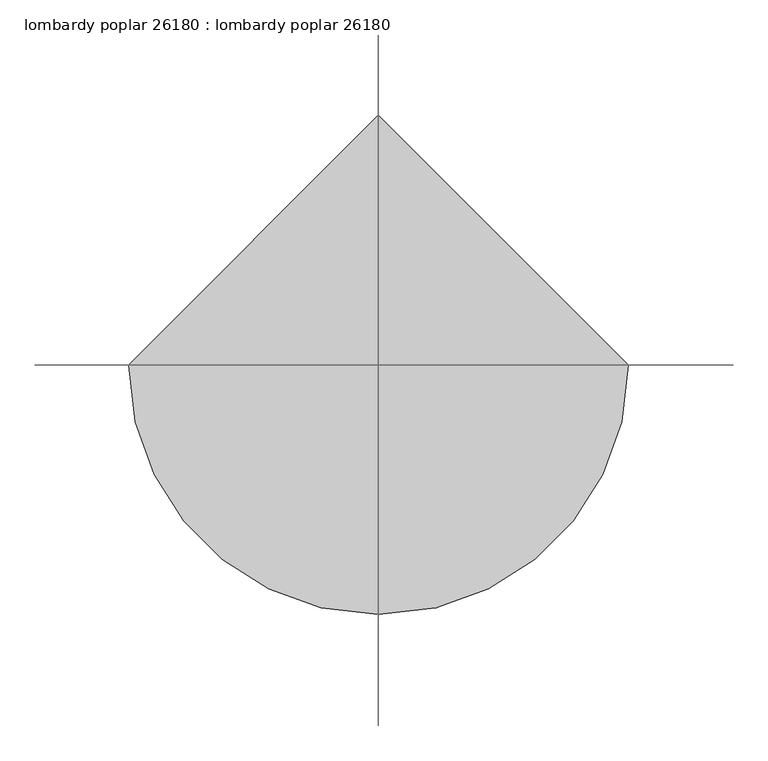
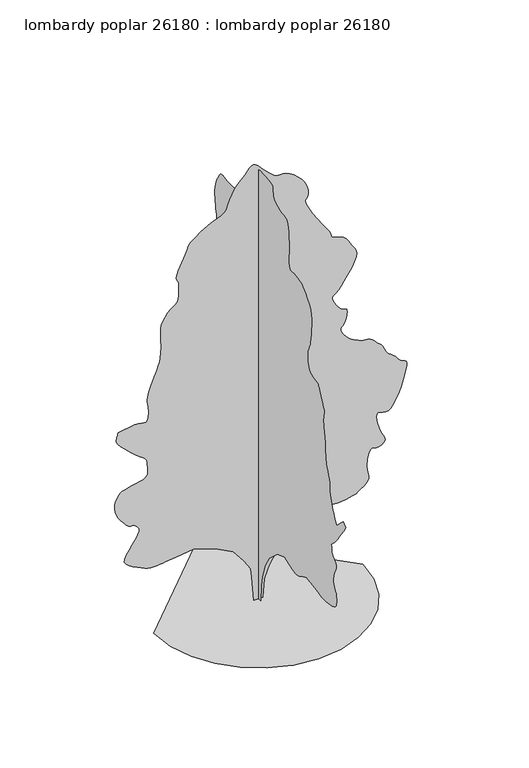
"""IFC4 building model written with IfcOpenShell, lengths in millimetres: proxy geometry, lombardy poplar 26180 : lombardy poplar 26180."""

import ifcopenshell
import ifcopenshell.guid

model = None  # the IFC model being written
_history = None  # IfcOwnerHistory: only IFC2X3 demands one
_inside = {}  # id of a spatial element -> (the spatial element, [elements in it])
_under = {}  # id of a project, library or spatial element -> (it, [spatial elements below it])
_declared = {}  # id of a project -> (the project, [libraries it declares])
_typed = {}  # id of a type object -> (the type object, [elements of that type])
_made_of = {}  # id of a material, layer set ... -> (it, [elements and type objects made of it])


def new_model(schema):
    """Start an empty IFC model of exactly this schema.

    Asked for "IFC4X3", IfcOpenShell would pick the latest addendum, in which some entities
    have other attributes; the version numbers below select the first issue.
    IFC2X3 requires an IfcOwnerHistory on every rooted entity: one is made here for all.
    """
    global model, _history
    if schema == "IFC4X3":
        model = ifcopenshell.file(schema_version=(4, 3, 0, 0))
    else:
        model = ifcopenshell.file(schema=schema)
    _inside.clear()
    _under.clear()
    _declared.clear()
    _typed.clear()
    _made_of.clear()
    _history = None
    if model.schema == "IFC2X3":
        org = make("IfcOrganization", Name="unknown")
        user = make(
            "IfcPersonAndOrganization",
            ThePerson=make("IfcPerson", FamilyName="unknown"),
            TheOrganization=org,
        )
        app = make(
            "IfcApplication",
            ApplicationDeveloper=org,
            Version="unknown",
            ApplicationFullName="unknown",
            ApplicationIdentifier="unknown",
        )
        _history = make(
            "IfcOwnerHistory",
            OwningUser=user,
            OwningApplication=app,
            ChangeAction="ADDED",
            CreationDate=0,
        )
    return model


def make(cls, **values):
    """One entity of the class cls with the attributes given. An attribute that is None is left unset."""
    return model.create_entity(
        cls, **{name: value for name, value in values.items() if value is not None}
    )


def rooted(cls, **values):
    """An entity with a GlobalId (a new one), such as an element, a storey or a relation."""
    return make(cls, GlobalId=ifcopenshell.guid.new(), OwnerHistory=_history, **values)


def si_unit(unit_type, name, prefix=None):
    """IfcSIUnit, for example si_unit("LENGTHUNIT", "METRE", prefix="MILLI")."""
    return make("IfcSIUnit", UnitType=unit_type, Prefix=prefix, Name=name)


def assignment(units):
    """IfcUnitAssignment: the units of a project."""
    return None if units is None else make("IfcUnitAssignment", Units=units)


def point(xyz):
    """IfcCartesianPoint."""
    return None if xyz is None else make("IfcCartesianPoint", Coordinates=xyz)


def direction(xyz):
    """IfcDirection."""
    return None if xyz is None else make("IfcDirection", DirectionRatios=xyz)


def frame(location, z_axis=None, x_axis=None):
    """IfcAxis2Placement3D, a coordinate frame: its origin and axes. An axis left out is left unset."""
    return make(
        "IfcAxis2Placement3D",
        Location=point(location),
        Axis=direction(z_axis),
        RefDirection=direction(x_axis),
    )


def origin():
    """The frame at (0, 0, 0) with its axes left unset."""
    return frame((0.0, 0.0, 0.0))


def place(relative_to, where):
    """IfcLocalPlacement: puts the frame where relative to a parent placement (None: the world)."""
    return make(
        "IfcLocalPlacement", PlacementRelTo=relative_to, RelativePlacement=where
    )


def context(
    kind, dimensions, precision=None, world=None, true_north=None, identifier=None
):
    """IfcGeometricRepresentationContext, for example the 3D "Model" context."""
    return make(
        "IfcGeometricRepresentationContext",
        ContextIdentifier=identifier,
        ContextType=kind,
        CoordinateSpaceDimension=dimensions,
        Precision=precision,
        WorldCoordinateSystem=world,
        TrueNorth=true_north,
    )


def project(units=None, contexts=None):
    """IfcProject with its units and contexts."""
    return rooted(
        "IfcProject",
        Name="project",
        RepresentationContexts=contexts,
        UnitsInContext=assignment(units),
    )


def spatial(cls, under=None, at=None, **own):
    """A site, building, storey or space (cls), placed at a placement, below another one or the project."""
    s = rooted(cls, ObjectPlacement=at, **own)
    if under is not None:
        _under.setdefault(under.id(), (under, []))[1].append(s)
    return s


def point_list(points):
    """IfcCartesianPointList2D or 3D."""
    cls = (
        "IfcCartesianPointList2D" if len(points[0]) == 2 else "IfcCartesianPointList3D"
    )
    return make(cls, CoordList=points)


def triangles(points, corners, closed=None, point_numbers=None):
    """IfcTriangulatedFaceSet: each triangle names its three corners, points numbered from 1."""
    return make(
        "IfcTriangulatedFaceSet",
        Coordinates=point_list(points),
        Closed=closed,
        CoordIndex=corners,
        PnIndex=point_numbers,
    )


def shape(context_of_items, identifier, shape_type, items):
    """IfcShapeRepresentation: the items that make up one representation, for example the "Body"."""
    return make(
        "IfcShapeRepresentation",
        ContextOfItems=context_of_items,
        RepresentationIdentifier=identifier,
        RepresentationType=shape_type,
        Items=items,
    )


def source(mapping_origin, context_of_items, identifier, shape_type, items):
    """IfcRepresentationMap: a shape defined once, which mapped items show again and again."""
    return make(
        "IfcRepresentationMap",
        MappingOrigin=mapping_origin,
        MappedRepresentation=shape(context_of_items, identifier, shape_type, items),
    )


def transform(
    local_origin,
    x_axis=None,
    y_axis=None,
    z_axis=None,
    scale=None,
    scale2=None,
    scale3=None,
    uniform=True,
):
    """IfcCartesianTransformationOperator3D, or its non-uniform kind. x_axis, y_axis, z_axis: its Axis1, 2, 3."""
    if uniform:
        return make(
            "IfcCartesianTransformationOperator3D",
            Axis1=direction(x_axis),
            Axis2=direction(y_axis),
            LocalOrigin=point(local_origin),
            Scale=scale,
            Axis3=direction(z_axis),
        )
    return make(
        "IfcCartesianTransformationOperator3DnonUniform",
        Axis1=direction(x_axis),
        Axis2=direction(y_axis),
        LocalOrigin=point(local_origin),
        Scale=scale,
        Axis3=direction(z_axis),
        Scale2=scale2,
        Scale3=scale3,
    )


def mapped(mapping_source, mapping_target):
    """IfcMappedItem: shows the shape of a source again, moved by a transform."""
    return make(
        "IfcMappedItem", MappingSource=mapping_source, MappingTarget=mapping_target
    )


def made_of(thing, what):
    """Note that an element or type object is made of a material, layer set ...; save() writes the relation."""
    if what is not None:
        _made_of.setdefault(what.id(), (what, []))[1].append(thing)
    return thing


def element(
    cls,
    number,
    at=None,
    inside=None,
    cuts=None,
    type_object=None,
    material=None,
    context=None,
    identifier="Body",
    shape_type=None,
    held_by="IfcProductDefinitionShape",
    body=None,
    shapes=None,
    **own,
):
    """One element of the class cls, such as IfcWall. Its Tag is "e" and its number.

    at: its placement. inside: the storey or other place that contains it. cuts: it is an
    opening in that element (IfcRelVoidsElement). A single representation is given by context,
    identifier, shape_type and body (its items); several are given by shapes. held_by: the class
    of the entity that holds the representations. save() writes the other relations.
    """
    e = rooted(cls, Tag="e%d" % number, ObjectPlacement=at, **own)
    if body is not None:
        shapes = [shape(context, identifier, shape_type, body)]
    if shapes is not None:
        e.Representation = make(held_by, Representations=shapes)
    if inside is not None:
        _inside.setdefault(inside.id(), (inside, []))[1].append(e)
    if cuts is not None:
        rooted(
            "IfcRelVoidsElement", RelatingBuildingElement=cuts, RelatedOpeningElement=e
        )
    if type_object is not None:
        _typed.setdefault(type_object.id(), (type_object, []))[1].append(e)
    return made_of(e, material)


def aggregate(whole, parts):
    """IfcRelAggregates: a whole, such as a stair, and the parts it consists of."""
    return rooted("IfcRelAggregates", RelatingObject=whole, RelatedObjects=parts)


def save(model, path):
    """Write the relations noted so far, then the file.

    IfcRelAggregates (storeys below a building ...), IfcRelContainedInSpatialStructure (elements
    in a storey), IfcRelDefinesByType, IfcRelAssociatesMaterial and IfcRelDeclares: one each for
    every whole, place, type object, material and project.
    """
    for whole, parts in _under.values():
        aggregate(whole, parts)
    for where, things in _inside.values():
        rooted(
            "IfcRelContainedInSpatialStructure",
            RelatedElements=things,
            RelatingStructure=where,
        )
    for kind, things in _typed.values():
        rooted("IfcRelDefinesByType", RelatedObjects=things, RelatingType=kind)
    for what, things in _made_of.values():
        rooted("IfcRelAssociatesMaterial", RelatedObjects=things, RelatingMaterial=what)
    for by, libraries in _declared.values():
        rooted("IfcRelDeclares", RelatingContext=by, RelatedDefinitions=libraries)
    model.write(path)


def lombardy_poplar_26180_lombardy_poplar_26180_01077960(model_context):
    return source(origin(), model_context, "Body", "Tessellation", [
        triangles([(0.0009695, 113.8156909, 0.0), (0.0009695, -104.8345258, 0.0), (0.0009695, -123.055434, 437.3009239), (0.0009695, -177.7179314, 728.8340738), (0.0009695, -323.483707, 1129.6911467), (0.0009695, -505.6928613, 1439.4461494), (0.0009695, -870.1086628, 1767.420607), (0.0009695, -1216.3049732, 1894.9664555), (0.0009695, -1398.5142002, 1822.0838402), (0.0009695, -1476.390406, 1795.1523445), (0.0009695, -1552.9941605, 1770.6083485), (0.0009695, -1627.0451637, 1750.8472), (0.0009695, -1697.2735806, 1738.2588696), (0.0009695, -1762.3991112, 1735.2286766), (0.0009695, -1821.1516296, 1744.1542946), (0.0009695, -1872.2563591, 1767.420607), (0.0009695, -1919.1091679, 1797.0624023), (0.0009695, -1965.9644474, 1823.8364948), (0.0009695, -2012.8172562, 1848.2204716), (0.0009695, -2059.6700649, 1870.6891582), (0.0009695, -2106.5227283, 1891.7279903), (0.0009695, -2153.3780079, 1911.8067066), (0.0009695, -2200.2308167, 1931.4103065), (0.0009695, -2582.8711235, 1876.7470734), (0.0009695, -2649.2156204, 1861.2353748), (0.0009695, -2715.4080917, 1846.3611374), (0.0009695, -2781.27006, 1832.7619675), (0.0009695, -2846.6750793, 1821.0754715), (0.0009695, -2911.4196739, 1811.9366398), (0.0009695, -2975.3765259, 1805.987875), (0.0009695, -3038.3939003, 1803.8619873), (0.0009695, -3111.6472778, 1806.252103), (0.0009695, -3200.5217949, 1814.0625275), (0.0009695, -3296.0764275, 1828.2459641), (0.0009695, -3389.4213112, 1849.7596218), (0.0009695, -3471.5901329, 1879.5614365), (0.0009695, -3533.6930283, 1918.6062916), (0.0009695, -3566.7892639, 1967.8516869), (0.0009695, -3579.2353065, 2021.4507408), (0.0009695, -3585.9154221, 2073.1371208), (0.0009695, -3587.8205383, 2123.2333363), (0.0009695, -3585.9154221, 2172.0521587), (0.0009695, -3581.1401321, 2219.915807), (0.0009695, -3574.4347275, 2267.139378), (0.0009695, -3566.7892639, 2314.0455265), (0.0009695, -3532.0422569, 2353.5170998), (0.0009695, -3499.7078934, 2395.5361919), (0.0009695, -3472.1235306, 2442.6555542), (0.0009695, -3451.7273918, 2497.4231415), (0.0009695, -3440.907122, 2562.3988266), (0.0009695, -3441.9992065, 2640.0972816), (0.0009695, -3457.4677391, 2733.1372421), (0.0009695, -3484.5187042, 2825.1865654), (0.0009695, -3515.3799019, 2900.6752716), (0.0009695, -3544.9708282, 2963.0830902), (0.0009695, -3568.1862717, 3015.940329), (0.0009695, -3579.9210205, 3062.7525879), (0.0009695, -3575.0695724, 3106.9993057), (0.0009695, -3548.5775848, 3152.2110809), (0.0009695, -3509.7918709, 3193.1050964), (0.0009695, -3472.6063499, 3225.0836678), (0.0009695, -3438.6212151, 3252.6171616), (0.0009695, -3409.3857903, 3280.1253662), (0.0009695, -3386.5511375, 3312.1039375), (0.0009695, -3371.6668716, 3352.997953), (0.0009695, -3366.3581841, 3407.3030685), (0.0009695, -3362.7005585, 3460.5158089), (0.0009695, -3354.9027786, 3498.4634926), (0.0009695, -3347.7145546, 3525.8699593), (0.0009695, -3345.9620453, 3547.5360786), (0.0009695, -3354.4202499, 3568.2624298), (0.0009695, -3377.8388786, 3592.7987228), (0.0009695, -3421.0188011, 3625.9458275), (0.0009695, -3481.5215034, 3679.8698616), (0.0009695, -3552.5654228, 3760.5655174), (0.0009695, -3632.3465996, 3863.5624283), (0.0009695, -3719.1381042, 3984.4155167), (0.0009695, -3811.2130074, 4118.6541252), (0.0009695, -3906.7676399, 4261.8084686), (0.0009695, -4004.1003616, 4409.432888), (0.0009695, -3894.7788368, 4518.779702), (0.0009695, -3749.0086647, 4391.221209), (0.0009695, -3603.2382019, 4227.2390671), (0.0009695, -3579.7434151, 4258.785688), (0.0009695, -3555.9689941, 4292.2630051), (0.0009695, -3531.5088593, 4329.5499733), (0.0009695, -3506.1342453, 4372.5775795), (0.0009695, -3479.4643616, 4423.2506493), (0.0009695, -3451.1939941, 4483.4992973), (0.0009695, -3421.0188011, 4555.2033508), (0.0009695, -3390.0055779, 4628.5837555), (0.0009695, -3360.2623352, 4695.8683113), (0.0009695, -3333.0587631, 4762.2383881), (0.0009695, -3309.6910034, 4832.7233299), (0.0009695, -3291.4028755, 4912.4536377), (0.0009695, -3279.5158104, 5006.5351044), (0.0009695, -3275.248629, 5120.0473618), (0.0009695, -3267.0697678, 5234.8554703), (0.0009695, -3245.5050957, 5333.3820145), (0.0009695, -3215.0252701, 5421.7481323), (0.0009695, -3180.0747871, 5505.9238083), (0.0009695, -3145.0993057, 5592.0551788), (0.0009695, -3114.6191895, 5686.1110657), (0.0009695, -3093.0545174, 5794.238768), (0.0009695, -3079.5672592, 5892.1298859), (0.0009695, -3069.8899429, 5959.4403122), (0.0009695, -3063.4130127, 6007.9286316), (0.0009695, -3059.4760437, 6049.4319122), (0.0009695, -3057.4691895, 6095.6854843), (0.0009695, -3056.7073174, 6158.5246719), (0.0009695, -3056.6055794, 6249.735965), (0.0009695, -3052.5671631, 6343.1320084), (0.0009695, -3042.1532639, 6412.2958099), (0.0009695, -3027.9291321, 6468.709227), (0.0009695, -3012.4097305, 6523.8523727), (0.0009695, -2998.1858894, 6589.2065231), (0.0009695, -2987.7716995, 6676.2017944), (0.0009695, -2983.7332832, 6796.3688782), (0.0009695, -2989.2957344, 6908.7381821), (0.0009695, -3001.5638809, 6976.78461), (0.0009695, -3013.8576073, 7018.6948425), (0.0009695, -3019.4200584, 7052.6288177), (0.0009695, -3011.6222786, 7096.7737976), (0.0009695, -2983.7332832, 7169.2908829), (0.0009695, -2929.0723755, 7288.340593), (0.0009695, -2866.7410057, 7418.1088348), (0.0009695, -2818.7857933, 7514.4256302), (0.0009695, -2782.7688057, 7582.8528488), (0.0009695, -2756.3021072, 7628.9541046), (0.0009695, -2737.0233421, 7658.3418457), (0.0009695, -2722.5201576, 7676.5535248), (0.0009695, -2710.4043274, 7689.2027527), (0.0009695, -2636.5666832, 7701.2421341), (0.0009695, -2564.8117607, 7715.3901077), (0.0009695, -2497.1818771, 7733.6523651), (0.0009695, -2435.7748695, 7758.1380798), (0.0009695, -2382.6507866, 7790.9296829), (0.0009695, -2339.8900246, 7834.0584457), (0.0009695, -2309.5548122, 7889.6335419), (0.0009695, -2289.3160767, 7951.0257248), (0.0009695, -2274.8152176, 8010.5377899), (0.0009695, -2265.0921192, 8068.4243729), (0.0009695, -2259.1968395, 8125.0662643), (0.0009695, -2256.1691174, 8180.7425171), (0.0009695, -2255.0515984, 8235.7589264), (0.0009695, -2254.8940498, 8290.4707031), (0.0009695, -2285.970932, 8345.7405853), (0.0009695, -2316.0901691, 8404.491069), (0.0009695, -2344.2968777, 8470.25159), (0.0009695, -2369.6358833, 8546.5277481), (0.0009695, -2391.1521572, 8636.8495605), (0.0009695, -2407.8857288, 8744.6726303), (0.0009695, -2418.8812786, 8873.551973), (0.0009695, -2430.0903328, 9004.9206985), (0.0009695, -2443.8493767, 9121.3031296), (0.0009695, -2453.7833633, 9227.8303482), (0.0009695, -2453.5168098, 9329.5572784), (0.0009695, -2436.6765587, 9431.5888412), (0.0009695, -2396.8874176, 9539.0561188), (0.0009695, -2327.7766651, 9657.0390335), (0.0009695, -2247.8811058, 9768.2398041), (0.0009695, -2177.228587, 9854.8798645), (0.0009695, -2111.6764835, 9921.4269653), (0.0009695, -2047.0792637, 9972.3796692), (0.0009695, -1979.2969185, 10012.156311), (0.0009695, -1904.1815907, 10045.2519653), (0.0009695, -1817.5931259, 10076.1128723), (0.0009695, -1725.5334835, 10094.8326599), (0.0009695, -1638.891679, 10096.3058258), (0.0009695, -1560.8554539, 10092.3688568), (0.0009695, -1494.6124043, 10094.8326599), (0.0009695, -1443.3501263, 10115.4325653), (0.0009695, -1410.2540359, 10166.0038971), (0.0009695, -1398.5142002, 10258.3319824), (0.0009695, -1400.4267288, 10362.6756134), (0.0009695, -1404.8895378, 10448.1971375), (0.0009695, -1409.9898079, 10525.1087219), (0.0009695, -1413.8125397, 10603.619046), (0.0009695, -1414.4501461, 10693.9414398), (0.0009695, -1409.9898079, 10806.2345856), (0.0009695, -1398.5142002, 10950.7350677), (0.0009695, -1382.6849339, 11097.4458801), (0.0009695, -1365.5779839, 11211.9737732), (0.0009695, -1345.9235149, 11297.8255096), (0.0009695, -1322.4438435, 11358.4811096), (0.0009695, -1293.8637566, 11397.4694275), (0.0009695, -1258.9083321, 11418.297226), (0.0009695, -1216.3049732, 11424.470105), (0.0009695, -1155.4822323, 11429.9813965), (0.0009695, -1073.3006933, 11446.3641174), (0.0009695, -979.6484882, 11473.2380585), (0.0009695, -884.3986336, 11510.3218414), (0.0009695, -797.4393339, 11557.2608368), (0.0009695, -728.6460766, 11613.8015717), (0.0009695, -687.9020519, 11679.5615112), (0.0009695, -672.8677952, 11749.3607391), (0.0009695, -668.0341513, 11816.289212), (0.0009695, -663.5180752, 11877.4785004), (0.0009695, -649.4413908, 11930.0811035), (0.0009695, -615.9210531, 11971.2041748), (0.0009695, -553.0790314, 11997.9757965), (0.0009695, -451.0296281, 12007.5263763), (0.0009695, -327.7864603, 12011.2087097), (0.0009695, -210.2816959, 12019.0070709), (0.0009695, -102.0189364, 12026.1694244), (0.0009695, -6.5056406, 12027.9216431), (0.0009695, 72.7523407, 12019.4895996), (0.0009695, 132.2489498, 11996.0700989), (0.0009695, 168.4781792, 11952.8657593), (0.0009695, 190.2581361, 11903.7920105), (0.0009695, 211.0820467, 11861.400412), (0.0009695, 234.4553475, 11819.0076508), (0.0009695, 263.8852554, 11769.9094849), (0.0009695, 302.8767344, 11707.4505066), (0.0009695, 354.9364746, 11624.9008942), (0.0009695, 423.5697126, 11515.57966), (0.0009695, 499.5867296, 11399.1204895), (0.0009695, 572.09851, 11297.9778259), (0.0009695, 642.0601553, 11209.5867096), (0.0009695, 710.4292379, 11131.3798553), (0.0009695, 778.1582434, 11060.8446259), (0.0009695, 846.2072874, 10995.3881561), (0.0009695, 915.531399, 10932.4978088), (0.0009695, 983.7404623, 10880.5556305), (0.0009695, 1048.444289, 10847.0786041), (0.0009695, 1110.5954372, 10828.282077), (0.0009695, 1171.1565662, 10820.3069824), (0.0009695, 1231.077618, 10819.3407623), (0.0009695, 1291.3160923, 10821.5766724), (0.0009695, 1352.8322502, 10823.1765747), (0.0009695, 1419.1287849, 10828.7646057), (0.0009695, 1490.5254444, 10841.0324615), (0.0009695, 1563.194846, 10853.3014801), (0.0009695, 1633.3164379, 10858.8639313), (0.0009695, 1697.0626923, 10851.0655701), (0.0009695, 1750.6084064, 10823.1765747), (0.0009695, 1790.1333195, 10768.5159576), (0.0009695, 1824.1844387, 10700.9526398), (0.0009695, 1861.7408672, 10636.2333344), (0.0009695, 1899.617189, 10570.5745514), (0.0009695, 1934.6234825, 10500.1404785), (0.0009695, 1963.5743317, 10421.0953033), (0.0009695, 1983.2847565, 10329.6299561), (0.0009695, 1990.5617832, 10221.8830444), (0.0009695, 1988.4357502, 10111.0130676), (0.0009695, 1982.4871307, 10010.9877777), (0.0009695, 1973.3507698, 9919.2433777), (0.0009695, 1961.6642738, 9833.2381622), (0.0009695, 1948.0651039, 9750.4350769), (0.0009695, 1933.1908665, 9668.2656738), (0.0009695, 1917.6791679, 9584.1667374), (0.0009695, 1914.3314072, 9505.3761978), (0.0009695, 1931.0649788, 9438.0663528), (0.0009695, 1961.1842159, 9378.0967575), (0.0009695, 1997.9989746, 9321.3025497), (0.0009695, 2034.813588, 9263.5682831), (0.0009695, 2064.9328251, 9200.7290955), (0.0009695, 2081.6663967, 9128.6439606), (0.0009695, 2081.1888096, 9058.6668365), (0.0009695, 2066.6854797, 9001.7964706), (0.0009695, 2041.9840805, 8953.1808334), (0.0009695, 2010.9071983, 8908.0707962), (0.0009695, 1977.2826519, 8861.6904877), (0.0009695, 1944.9307022, 8809.2646179), (0.0009695, 1917.6791679, 8745.9934799), (0.0009695, 1901.8472855, 8673.7048691), (0.0009695, 1900.361475, 8598.2164536), (0.0009695, 1911.9412914, 8520.8229218), (0.0009695, 1935.3142834, 8442.7939636), (0.0009695, 1969.2055286, 8365.374852), (0.0009695, 2012.3422852, 8289.8864365), (0.0009695, 2063.4443985, 8217.5978256), (0.0009695, 2116.1951031, 8158.060762), (0.0009695, 2166.3955273, 8113.7884644), (0.0009695, 2215.9584904, 8075.6123062), (0.0009695, 2266.796521, 8034.2101822), (0.0009695, 2320.8222931, 7980.4134659), (0.0009695, 2379.9457191, 7904.924469), (0.0009695, 2446.0820892, 7798.5239868), (0.0009695, 2515.4595406, 7684.1478287), (0.0009695, 2583.8870499, 7588.5931961), (0.0009695, 2652.6194824, 7508.3039108), (0.0009695, 2722.9518173, 7439.8511124), (0.0009695, 2796.1546165, 7379.653624), (0.0009695, 2873.4972794, 7324.2558426), (0.0009695, 2956.2759476, 7270.103334), (0.0009695, 3039.9940933, 7227.3042023), (0.0009695, 3119.5720848, 7202.0063278), (0.0009695, 3195.3148453, 7185.0137604), (0.0009695, 3267.5522964, 7167.0555542), (0.0009695, 3336.6149414, 7138.9125046), (0.0009695, 3402.807122, 7091.3130844), (0.0009695, 3466.4593414, 7015.0113464), (0.0009695, 3525.2604034, 6921.5903046), (0.0009695, 3575.4506538, 6829.7441666), (0.0009695, 3615.1508469, 6741.0728348), (0.0009695, 3642.3797081, 6657.2023727), (0.0009695, 3655.3082794, 6579.6815231), (0.0009695, 3651.9552864, 6510.1619293), (0.0009695, 3630.4414833, 6450.1673355), (0.0009695, 3590.004998, 6392.5348068), (0.0009695, 3534.6075073, 6330.4316208), (0.0009695, 3469.3295151, 6266.1192673), (0.0009695, 3399.2512344, 6201.7813339), (0.0009695, 3329.5028755, 6139.6781479), (0.0009695, 3265.1646515, 6082.0456192), (0.0009695, 3211.3676445, 6031.0934967), (0.0009695, 3161.7869499, 5985.0939789), (0.0009695, 3109.3613708, 5939.7298874), (0.0009695, 3057.8758507, 5893.4001572), (0.0009695, 3011.1906189, 5844.5304657), (0.0009695, 2973.1159081, 5791.5209106), (0.0009695, 2947.4366615, 5732.7710083), (0.0009695, 2938.0386887, 5666.680275), (0.0009695, 2934.1778778, 5597.4141541), (0.0009695, 2924.8816429, 5529.7235184), (0.0009695, 2913.6547119, 5463.0235199), (0.0009695, 2904.0535538, 5396.6025742), (0.0009695, 2899.5323181, 5329.8764145), (0.0009695, 2903.6218941, 5262.2113586), (0.0009695, 2919.8270096, 5192.9452377), (0.0009695, 2944.8458313, 5126.3719757), (0.0009695, 2972.7351173, 5066.5046997), (0.0009695, 3003.0117577, 5012.2248734), (0.0009695, 3035.1935143, 4962.3901245), (0.0009695, 3068.8231476, 4915.908078), (0.0009695, 3103.4178383, 4871.6613602), (0.0009695, 3138.4697685, 4828.5323067), (0.0009695, 3181.1415825, 4835.3141602), (0.0009695, 3222.035598, 4836.0760323), (0.0009695, 3259.4243042, 4824.696785), (0.0009695, 3291.5807716, 4795.1567276), (0.0009695, 3316.7013313, 4741.4102989), (0.0009695, 3333.0587631, 4657.3619408), (0.0009695, 3338.9008484, 4536.9916718), (0.0009695, 3338.9008484, 3935.6984322), (0.0009695, 3345.6065437, 3757.6444748), (0.0009695, 3361.2273926, 3611.1377197), (0.0009695, 3379.0582809, 3492.0371407), (0.0009695, 3392.4440918, 3396.2031647), (0.0009695, 3394.6791298, 3319.4953468), (0.0009695, 3379.0582809, 3257.747953), (0.0009695, 3338.9008484, 3206.8719887), (0.0009695, 3281.573243, 3178.2461197), (0.0009695, 3221.7053856, 3174.1568344), (0.0009695, 3163.4380119, 3176.747374), (0.0009695, 3110.9106949, 3168.187722), (0.0009695, 3068.2388809, 3130.6466995), (0.0009695, 3039.6130119, 3046.21726), (0.0009695, 3029.1482437, 2897.119384), (0.0009695, 3036.0571243, 2732.8070297), (0.0009695, 3053.1514297, 2608.9823204), (0.0009695, 3075.0460236, 2517.0268867), (0.0009695, 3096.3057724, 2448.3400909), (0.0009695, 3111.4949615, 2394.3144642), (0.0009695, 3115.2034561, 2346.3441364), (0.0009695, 3102.0208305, 2295.8261444), (0.0009695, 3089.0669701, 2254.1778145), (0.0009695, 3089.803553, 2232.6106716), (0.0009695, 3093.4355988, 2222.1992432), (0.0009695, 3089.0669701, 2214.0179111), (0.0009695, 3065.9021049, 2199.1436737), (0.0009695, 3013.0954445, 2168.6510582), (0.0009695, 2919.8270096, 2113.6169174), (0.0009695, 2822.3419716, 2052.8450455), (0.0009695, 2753.55867, 2008.9666191), (0.0009695, 2697.5010452, 1978.7940422), (0.0009695, 2638.2683235, 1959.1395733), (0.0009695, 2559.9350235, 1946.8154709), (0.0009695, 2446.5088074, 1938.6341389), (0.0009695, 2282.0948605, 1931.4103065), (0.0009695, 2105.8903542, 1933.6938881), (0.0009695, 1963.4702682, 1951.9132702), (0.0009695, 1848.4591198, 1979.6982021), (0.0009695, 1754.4869488, 2010.665934), (0.0009695, 1675.1755108, 2038.4483952), (0.0009695, 1604.1522297, 2056.670248), (0.0009695, 1535.0414772, 2058.9536842), (0.0009695, 1460.510416, 2049.0198429), (0.0009695, 1378.3312752, 2035.2631245), (0.0009695, 1289.7769421, 2018.3163391), (0.0009695, 1196.1221935, 1998.8218895), (0.0009695, 1098.6447859, 1977.4122952), (0.0009695, 998.6146271, 1954.7301041), (0.0009695, 897.3120169, 1931.4103065), (0.0009695, 532.8936719, 1639.8747585), (0.0009695, 314.2457534, 1166.1349977), (0.0009695, 168.4781792, 601.2881527), (120.1776209, 0.0005334, 0.0085345), (-116.69275, 0.0005334, 0.0085345), (-171.3552383, 0.0004849, 655.9590162), (-207.7973272, 0.0004849, 911.0508585), (-390.006209, 0.0004607, 1202.5839357), (-663.3174334, 0.0004364, 1548.7803188), (-1137.0596649, 0.0004122, 1803.8721611), (-1720.1284355, 0.0004122, 1986.078772), (-2193.8681236, 0.0004122, 1931.4180096), (-2467.1819641, 0.0004122, 1894.9766293), (-2533.7959213, 0.0004122, 1885.46689), (-2607.4327057, 0.0004122, 1874.6820831), (-2686.1473778, 0.0004122, 1865.812421), (-2768.0621452, 0.0004122, 1862.0405582), (-2851.2468933, 0.0004122, 1866.556707), (-2933.7967964, 0.0004122, 1882.5459927), (-3013.8067383, 0.0004122, 1913.1960114), (-3104.2814484, 0.0004122, 1955.5886272), (-3210.9865631, 0.0004122, 2004.6715324), (-3321.222567, 0.0004122, 2060.4522846), (-3422.2126236, 0.0004122, 2122.9234715), (-3501.2066391, 0.0003879, 2192.0875637), (-3545.4533569, 0.0003879, 2267.9445614), (-3542.2021019, 0.0003879, 2350.4969353), (-3495.1869484, 0.0003879, 2447.2326004), (-3424.930481, 0.0003879, 2559.9094437), (-3343.8031654, 0.0003637, 2679.898922), (-3264.2757523, 0.0003637, 2798.6437088), (-3198.7692856, 0.0003637, 2907.4824142), (-3159.7295174, 0.0003394, 2997.8300972), (-3159.5772011, 0.0003394, 3061.1015259), (-3182.9958298, 0.0003394, 3103.1893639), (-3206.4147491, 0.0003394, 3136.6411011), (-3229.8589577, 0.0003394, 3162.9554832), (-3253.2775864, 0.0003394, 3183.5039383), (-3276.6962151, 0.0003394, 3199.7599228), (-3300.1404236, 0.0003394, 3213.1457336), (-3323.559343, 0.0003394, 3225.1089569), (-3347.1558678, 0.0003394, 3221.5783585), (-3371.6921608, 0.0003394, 3220.486274), (-3398.1335701, 0.0003394, 3224.1438995), (-3427.4704422, 0.0003394, 3234.9897491), (-3460.6175468, 0.0003394, 3255.3858879), (-3498.5396507, 0.0003394, 3287.7199608), (-3542.2021019, 0.0003394, 3334.4304817), (-3593.6370438, 0.0003394, 3395.5174507), (-3650.1519081, 0.0003152, 3468.3897469), (-3705.7270042, 0.0003152, 3551.4730476), (-3754.2664833, 0.0003152, 3643.1668694), (-3789.7500732, 0.0003152, 3741.8713097), (-3806.1330849, 0.0002909, 3845.9855942), (-3797.2937988, 0.0002909, 3953.9354004), (-3771.4366562, 0.0002909, 4051.5730453), (-3739.8138771, 0.0002909, 4128.1791252), (-3701.2057686, 0.0002909, 4187.2342415), (-3654.2920624, 0.0002667, 4232.2937004), (-3597.828067, 0.0002667, 4266.812233), (-3530.518222, 0.0002667, 4294.3457268), (-3451.117836, 0.0002667, 4318.3486221), (-3356.8078949, 0.0002667, 4338.3131012), (-3252.3378181, 0.0002667, 4355.4326958), (-3147.5122398, 0.0002667, 4375.7270966), (-3052.2622398, 0.0002667, 4405.2674446), (-2976.4689011, 0.0002667, 4450.0981384), (-2929.9868546, 0.0002667, 4516.2906097), (-2922.6971832, 0.0002667, 4609.8895477), (-2933.5936111, 0.0002425, 4707.6283493), (-2938.4197701, 0.0002425, 4784.9713028), (-2942.3058701, 0.0002425, 4846.0582718), (-2950.332415, 0.0002425, 4895.0291199), (-2967.578746, 0.0002425, 4936.0504532), (-2999.2018158, 0.0002425, 4973.2359741), (-3050.2556763, 0.0002425, 5010.7517075), (-3135.4978569, 0.0002182, 5072.041571), (-3254.8777794, 0.0002182, 5168.7141586), (-3391.1232422, 0.0002182, 5287.0778641), (-3527.0637817, 0.0002182, 5413.3916656), (-3645.4783562, 0.000194, 5533.9906998), (-3729.1459236, 0.000194, 5635.1333633), (-3760.8704407, 0.000194, 5703.129213), (-3759.2702477, 0.000194, 5747.3247711), (-3754.799881, 0.000194, 5786.7456207), (-3747.9418694, 0.000194, 5822.178923), (-3739.1787415, 0.0001697, 5854.4112579), (-3728.9933167, 0.0001697, 5884.2815277), (-3717.8428345, 0.0001697, 5912.5263153), (-3706.2095329, 0.0001697, 5940.0089401), (-3268.8984352, 0.0001697, 6012.8818176), (-3174.1312546, 0.0001697, 6014.48172), (-3093.0545174, 0.0001697, 5998.8605804), (-3026.0240158, 0.0001697, 5982.2743835), (-2973.319384, 0.0001697, 5981.0046936), (-2935.2955421, 0.0001697, 6011.2813339), (-2912.232415, 0.0001697, 6089.3864502), (-2904.4852135, 0.0001697, 6231.5242859), (-2910.9624344, 0.0001455, 6377.1421417), (-2925.0848282, 0.0001455, 6470.4870255), (-2938.9022987, 0.0001455, 6535.1301727), (-2944.4394608, 0.0001455, 6594.6678177), (-2933.6953491, 0.0001212, 6672.7217743), (-2898.7448662, 0.0001212, 6792.8126999), (-2831.5873375, 0.0001212, 6978.5879883), (-2754.346122, 9.7e-05, 7175.5649185), (-2693.3861801, 9.7e-05, 7325.0435852), (-2647.0567406, 9.7e-05, 7444.2456116), (-2613.8081886, 7.27e-05, 7550.3920395), (-2592.0150421, 7.27e-05, 7660.678331), (-2580.127977, 7.27e-05, 7792.3011108), (-2576.4956406, 4.85e-05, 7962.5064194), (-2580.0009499, 4.85e-05, 8135.9626923), (-2586.7063545, 4.85e-05, 8272.4363388), (-2590.8467995, 2.42e-05, 8381.8087326), (-2586.7063545, 2.42e-05, 8473.985083), (-2568.5455444, 2.42e-05, 8558.8211838), (-2530.6106506, 2.42e-05, 8646.1972458), (-2467.1819641, 0.0, 8746.0190598), (-2393.5550629, 0.0, 8838.8046753), (-2328.8511635, 0.0, 8903.8797729), (-2273.0728821, 0.0, 8949.1932861), (-2226.2200733, 0.0, 8982.7208908), (-2188.2902664, 0.0, 9012.4138458), (-2159.2860775, 0.0, 9046.2460831), (-2139.2048904, 0.0, 9092.1950226), (-2125.7124001, -2.42e-05, 9135.3493652), (-2116.0452576, -2.42e-05, 9162.8575699), (-2109.5630951, -2.42e-05, 9185.920697), (-2105.6338291, -2.42e-05, 9215.6642303), (-2103.6144756, -2.42e-05, 9263.2636505), (-2102.8701897, -2.42e-05, 9339.8700211), (-2102.7661263, -2.42e-05, 9456.6332428), (-2113.0708752, -4.85e-05, 9567.5549606), (-2136.1264446, -4.85e-05, 9634.4840149), (-2160.137043, -4.85e-05, 9680.3817947), (-2173.3094948, -4.85e-05, 9728.1846909), (-2163.855566, -4.85e-05, 9800.8540924), (-2119.9745235, -7.27e-05, 9921.3258087), (-2029.8808949, -7.27e-05, 10112.5618103), (-1939.4672276, -7.27e-05, 10305.830246), (-1888.8958958, -9.7e-05, 10431.5097839), (-1857.7656738, -9.7e-05, 10511.3165405), (-1825.6805683, -9.7e-05, 10566.8654755), (-1772.2389175, -9.7e-05, 10619.9006104), (-1677.0450188, -9.7e-05, 10692.0369049), (-1519.6973557, -0.0001212, 10804.9648956), (-1341.6868549, -0.0001212, 10917.309201), (-1195.5481733, -0.0001212, 10985.3806274), (-1077.4586517, -0.0001212, 11027.29086), (-983.5905441, -0.0001212, 11061.2248352), (-910.1237349, -0.0001212, 11105.3698151), (-853.2303326, -0.0001455, 11177.8874817), (-809.0852074, -0.0001455, 11296.9371918), (-759.9464916, -0.0001455, 11440.4714539), (-694.8717573, -0.0001697, 11572.8563965), (-620.2365601, -0.0001697, 11691.8293671), (-542.413585, -0.0001697, 11795.2079407), (-467.775808, -0.0001697, 11880.7294647), (-402.7036534, -0.0001697, 11946.1847717), (-353.5649014, -0.000194, 11989.3146973), (-315.2642959, -0.000194, 12029.8529205), (-276.9611651, -0.000194, 12081.541626), (-236.4299363, -0.000194, 12133.2303314), (-191.4351718, -0.000194, 12173.7685547), (-139.7475292, -0.000194, 12191.9802338), (-79.1353495, -0.000194, 12176.7404663), (-7.3676139, -0.000194, 12116.8731903), (68.4904824, -0.000194, 12035.3130524), (139.8862108, -0.000194, 11962.0605469), (206.8199341, -0.0001697, 11896.4517609), (269.290376, -0.0001697, 11837.8797546), (327.3013518, -0.0001697, 11785.6573608), (380.8469934, -0.0001697, 11739.1753143), (429.9324057, -0.0001697, 11697.7987701), (477.3160323, -0.0001697, 11672.4491547), (527.8899076, -0.0001697, 11666.8622864), (584.8366133, -0.0001697, 11669.5795624), (651.343891, -0.0001697, 11669.0970337), (730.6019165, -0.0001697, 11653.9584229), (825.7958879, -0.0001697, 11612.684198), (940.1160175, -0.0001455, 11533.7913391), (1053.1051964, -0.0001455, 11434.3508972), (1143.4680674, -0.0001455, 11338.4148926), (1213.1096741, -0.0001455, 11245.0194305), (1263.9477047, -0.0001455, 11153.2238708), (1297.8921444, -0.0001212, 11062.0631561), (1316.8558125, -0.0001212, 10970.5978088), (1322.7537083, -0.0001212, 10877.8371918), (1310.6404942, -0.0001212, 10807.3019623), (1283.8688725, -0.0001212, 10768.6426941), (1256.7747414, -0.0001212, 10740.1444336), (1243.7064983, -9.7e-05, 10700.2154755), (1259.0074539, -9.7e-05, 10627.1141235), (1317.0158318, -9.7e-05, 10499.1998383), (1432.0777039, -7.27e-05, 10294.7809204), (1568.3356659, -7.27e-05, 10074.4362305), (1681.0074223, -4.85e-05, 9906.365094), (1771.0503273, -4.85e-05, 9780.3565063), (1839.4167938, -4.85e-05, 9686.22388), (1887.067083, -4.85e-05, 9613.757373), (1914.9562237, -4.85e-05, 9552.772142), (1924.041861, -2.42e-05, 9493.0571823), (1943.5896503, -2.42e-05, 9444.2892288), (1995.6494087, -2.42e-05, 9415.2822784), (2070.3380184, -2.42e-05, 9394.5812164), (2157.7773033, -2.42e-05, 9370.6797684), (2248.0842911, -2.42e-05, 9332.0972397), (2331.3809509, -2.42e-05, 9267.4035141), (2397.7841652, -2.42e-05, 9165.0928986), (2454.6240097, 0.0, 9055.2379761), (2511.1467224, 0.0, 8968.9542892), (2560.341394, 0.0, 8896.3866257), (2595.190139, 0.0, 8827.6541931), (2608.6773972, 0.0, 8752.8512009), (2593.7931313, 2.42e-05, 8662.1230179), (2543.5520119, 2.42e-05, 8545.5876892), (2481.3447624, 2.42e-05, 8432.1260101), (2431.8886242, 2.42e-05, 8349.5508179), (2390.080275, 2.42e-05, 8286.457576), (2350.8220608, 4.85e-05, 8231.3138489), (2309.0163277, 4.85e-05, 8172.6656845), (2259.5600441, 4.85e-05, 8099.0312256), (2197.3530853, 4.85e-05, 7998.9553574), (2127.0206051, 4.85e-05, 7904.0355698), (2060.8307499, 7.27e-05, 7844.1677124), (2005.159148, 7.27e-05, 7805.3311295), (1966.378521, 7.27e-05, 7773.5051651), (1950.8666771, 7.27e-05, 7734.6685822), (1964.9992447, 7.27e-05, 7674.8007248), (2015.1464745, 7.27e-05, 7579.8815186), (2080.6452381, 7.27e-05, 7478.1545883), (2137.5387131, 9.7e-05, 7404.1387573), (2187.2590794, 9.7e-05, 7353.262793), (2231.2468014, 9.7e-05, 7320.852562), (2270.9265015, 9.7e-05, 7302.3106705), (2307.7412601, 9.7e-05, 7293.0141449), (2343.1207867, 9.7e-05, 7288.340593), (2346.839455, 9.7e-05, 7260.6544922), (2349.4429298, 9.7e-05, 7230.9109589), (2349.8136921, 9.7e-05, 7197.027562), (2346.839455, 9.7e-05, 7156.9212891), (2339.4022636, 9.7e-05, 7108.5341263), (2326.3873604, 0.0001212, 7049.7842239), (2306.6795517, 0.0001212, 6978.5879883), (2277.832766, 0.0001212, 6914.427951), (2243.2507198, 0.0001212, 6871.273027), (2210.5813477, 0.0001212, 6838.9901138), (2187.4724384, 0.0001212, 6807.3158844), (2181.5771587, 0.0001212, 6766.0922379), (2200.5406815, 0.0001212, 6705.1064255), (2252.0163185, 0.0001455, 6614.1747665), (2322.1379105, 0.0001455, 6519.5090332), (2391.3020027, 0.0001455, 6450.3452316), (2458.553421, 0.0001455, 6400.9424332), (2522.9372818, 0.0001455, 6365.5602905), (2583.5059685, 0.0001455, 6338.4584564), (2639.2842499, 0.0001455, 6313.9221634), (2689.322184, 0.0001455, 6286.184903), (2738.2427444, 0.0001455, 6263.7822006), (2790.6680328, 0.0001455, 6254.1048843), (2845.659153, 0.0001697, 6249.8632828), (2902.2248863, 0.0001697, 6243.6909851), (2959.4507538, 0.0001697, 6228.2989014), (3016.3466995, 0.0001697, 6196.3200394), (3071.9473755, 0.0001697, 6140.4403107), (3121.4519119, 0.0001697, 6084.0774719), (3162.3712166, 0.0001697, 6048.746489), (3197.2199615, 0.0001697, 6024.2607742), (3228.5633972, 0.0001697, 6000.4104858), (3258.9417755, 0.0001697, 5966.9840378), (3290.9203468, 0.0001697, 5913.8215851), (3327.0390724, 0.000194, 5830.687706), (3367.3235321, 0.000194, 5746.3091354), (3410.4525856, 0.000194, 5689.0573975), (3457.0869484, 0.000194, 5648.0366455), (3507.8614655, 0.000194, 5612.4510269), (3563.4365616, 0.000194, 5571.430275), (3624.4217926, 0.000194, 5514.178537), (3691.4522942, 0.0002182, 5429.8255463), (3759.9306725, 0.0002182, 5354.920816), (3822.0335678, 0.0002182, 5319.208461), (3873.620826, 0.0002182, 5301.6827866), (3910.5270035, 0.0002182, 5281.2863571), (3928.6625244, 0.0002182, 5236.989061), (3923.8110764, 0.0002182, 5147.7334625), (3891.883374, 0.0002425, 4992.5144485), (3839.8897453, 0.0002425, 4801.4304726), (3779.2600159, 0.0002667, 4621.8274818), (3712.6105957, 0.0002667, 4458.4801849), (3642.4302864, 0.0002667, 4316.1641624), (3571.3104996, 0.0002909, 4199.6799934), (3501.7653259, 0.0002909, 4113.777388), (3436.3605972, 0.0002909, 4063.2569252), (3368.5935127, 0.0002909, 4052.055574), (3295.6956367, 0.0002909, 4067.2956322), (3225.9981468, 0.0002909, 4088.6059593), (3167.7813515, 0.0002909, 4095.5657089), (3129.3258499, 0.0002909, 4067.7781609), (3118.9119507, 0.0002909, 3984.8471764), (3144.8452515, 0.0002909, 3826.3769073), (3196.8388802, 0.0003152, 3648.5264259), (3252.998243, 0.0003152, 3514.6686081), (3304.0521034, 0.0003152, 3415.2278755), (3340.7550957, 0.0003394, 3340.6280685), (3353.8615631, 0.0003394, 3281.3444778), (3334.1764275, 0.0003394, 3227.8015251), (3272.3784554, 0.0003394, 3170.4230507), (3191.911274, 0.0003394, 3134.2534561), (3121.6295174, 0.0003394, 3135.3711205), (3060.5934174, 0.0003394, 3150.839653), (3007.8379166, 0.0003394, 3157.6976646), (2962.4226654, 0.0003394, 3132.9834755), (2923.3828972, 0.0003394, 3053.7862747), (2889.7532639, 0.0003637, 2897.119384), (2876.0881096, 0.0003637, 2719.1165863), (2887.6196732, 0.0003879, 2584.1155243), (2909.3366615, 0.0003879, 2481.6546272), (2926.3039398, 0.0003879, 2401.1749466), (2923.4846352, 0.0003879, 2332.1708736), (2885.9180328, 0.0003879, 2264.1218296), (2798.6437088, 0.0003879, 2186.5098518), (2701.5906212, 0.0004122, 2115.113047), (2635.7792313, 0.0004122, 2068.2602383), (2587.7987297, 0.0004122, 2039.2560493), (2544.2885948, 0.0004122, 2021.4075748), (2491.8603996, 0.0004122, 2008.0191479), (2417.1185955, 0.0004122, 1992.4007698), (2306.6795517, 0.0004122, 1967.8592445), (2182.1079403, 0.0004122, 1946.8763683), (2070.9247559, 0.0004122, 1942.7844669), (1968.6644279, 0.0004122, 1950.1707893), (1870.8670544, 0.0004122, 1963.60994), (1773.0695354, 0.0004122, 1977.6865517), (1670.8093529, 0.0004122, 1986.9829319), (1559.6260231, 0.0004122, 1986.078772), (1454.709026, 0.0004122, 1976.1447853), (1371.7857445, 0.0004122, 1962.3882122), (1307.1885246, 0.0004122, 1945.4412815), (1257.2547993, 0.0004122, 1925.9468319), (1218.3166964, 0.0004122, 1904.5372375), (1186.70896, 0.0004122, 1881.8550465), (1158.7664795, 0.0004122, 1858.5353943), (1158.4464409, 0.0004364, 1761.2688023), (1156.2163445, 0.0004364, 1666.0722874), (1150.1584293, 0.0004364, 1575.0234844), (1138.3677246, 0.0004364, 1490.1876743), (1118.9240713, 0.0004364, 1413.6372597), (1089.9198824, 0.0004607, 1347.4475498), (1049.4399405, 0.0004607, 1293.6884766), (1004.179767, 0.0004607, 1251.6160446), (961.7897673, 0.0004607, 1218.1490467), (921.7874125, 0.0004607, 1191.8550121), (883.7001297, 0.0004607, 1171.2962379), (847.045463, 0.0004607, 1155.0403261), (811.3483686, 0.0004607, 1141.6519718), (776.1287888, 0.0004607, 1129.7013205), (466.3737496, 0.0004607, 1129.7013205), (284.1645772, 0.0004849, 856.3875526), (156.6199641, 0.0005092, 510.1912059), (-2766.0555817, 0.0, 0.0100862), (-2692.9292313, -633.8001217, 0.0100862), (-2484.680024, -1215.8427195, 0.0100862), (-2157.9602863, -1729.4553371, 0.0100862), (-1729.4553371, -2157.9602863, 0.0100862), (-1215.8427195, -2484.680024, 0.0100862), (-633.8001217, -2692.9292313, 0.0100862), (0.0001209, -2766.0555817, 0.0100862), (633.8001217, -2692.9292313, 0.0100862), (1215.8427195, -2484.680024, 0.0100862), (1729.4553371, -2157.9602863, 0.0100862), (2157.9602863, -1729.4553371, 0.0100862), (2484.680024, -1215.8427195, 0.0100862), (2692.9292313, -633.8001217, 0.0100862), (2766.0555817, 0.0002425, 0.0100862), (-0.0003627, 2766.0555817, 0.0100862)], [[1, 2, 3], [388, 1, 3], [388, 3, 4], [387, 388, 4], [387, 4, 5], [80, 81, 82], [79, 80, 82], [79, 82, 83], [78, 79, 83], [77, 78, 83], [387, 5, 6], [386, 387, 6], [76, 77, 83], [386, 6, 7], [359, 360, 361], [359, 361, 362], [385, 386, 7], [75, 76, 83], [75, 83, 84], [75, 84, 85], [74, 75, 85], [73, 74, 85], [73, 85, 86], [72, 73, 86], [72, 86, 87], [358, 359, 362], [358, 362, 363], [72, 87, 88], [131, 132, 133], [71, 72, 88], [130, 131, 133], [129, 130, 133], [71, 88, 89], [44, 45, 46], [128, 129, 133], [71, 89, 90], [207, 208, 209], [207, 209, 210], [206, 207, 210], [205, 206, 210], [205, 210, 211], [205, 211, 212], [204, 205, 212], [204, 212, 213], [203, 204, 213], [203, 213, 214], [203, 214, 215], [202, 203, 215], [202, 215, 216], [201, 202, 216], [200, 201, 216], [199, 200, 216], [198, 199, 216], [197, 198, 216], [196, 197, 216], [195, 196, 216], [194, 195, 216], [194, 216, 217], [193, 194, 217], [193, 217, 218], [193, 218, 219], [192, 193, 219], [192, 219, 220], [191, 192, 220], [191, 220, 221], [191, 221, 222], [190, 191, 222], [190, 222, 223], [128, 133, 134], [127, 128, 134], [71, 90, 91], [235, 236, 237], [234, 235, 237], [233, 234, 237], [233, 237, 238], [232, 233, 238], [232, 238, 239], [231, 232, 239], [231, 239, 240], [231, 240, 241], [231, 241, 242], [230, 231, 242], [230, 242, 243], [230, 243, 244], [230, 244, 245], [229, 230, 245], [229, 245, 246], [228, 229, 246], [228, 246, 247], [227, 228, 247], [227, 247, 248], [227, 248, 249], [226, 227, 249], [226, 249, 250], [226, 250, 251], [225, 226, 251], [225, 251, 252], [224, 225, 252], [71, 91, 92], [189, 190, 223], [330, 331, 332], [330, 332, 333], [329, 330, 333], [329, 333, 334], [328, 329, 334], [328, 334, 335], [328, 335, 336], [327, 328, 336], [385, 7, 8], [342, 343, 344], [341, 342, 344], [341, 344, 345], [340, 341, 345], [340, 345, 346], [339, 340, 346], [339, 346, 347], [338, 339, 347], [337, 338, 347], [337, 347, 348], [336, 337, 348], [327, 336, 348], [326, 327, 348], [325, 326, 348], [324, 325, 348], [323, 324, 348], [126, 127, 134], [126, 134, 135], [357, 358, 363], [357, 363, 364], [356, 357, 364], [355, 356, 364], [354, 355, 364], [353, 354, 364], [353, 364, 365], [352, 353, 365], [352, 365, 366], [352, 366, 367], [352, 367, 368], [352, 368, 369], [352, 369, 370], [351, 352, 370], [351, 370, 371], [351, 371, 372], [350, 351, 372], [350, 372, 373], [350, 373, 374], [350, 374, 375], [350, 375, 376], [349, 350, 376], [349, 376, 377], [348, 349, 377], [323, 348, 377], [323, 377, 378], [323, 378, 379], [323, 379, 380], [322, 323, 380], [322, 380, 381], [322, 381, 382], [321, 322, 382], [321, 382, 383], [321, 383, 384], [321, 384, 385], [321, 385, 8], [320, 321, 8], [319, 320, 8], [318, 319, 8], [317, 318, 8], [316, 317, 8], [315, 316, 8], [314, 315, 8], [313, 314, 8], [57, 58, 59], [56, 57, 59], [56, 59, 60], [55, 56, 60], [55, 60, 61], [54, 55, 61], [54, 61, 62], [53, 54, 62], [53, 62, 63], [53, 63, 64], [52, 53, 64], [36, 37, 38], [36, 38, 39], [35, 36, 39], [35, 39, 40], [35, 40, 41], [34, 35, 41], [34, 41, 42], [34, 42, 43], [33, 34, 43], [33, 43, 44], [33, 44, 46], [33, 46, 47], [32, 33, 47], [32, 47, 48], [31, 32, 48], [30, 31, 48], [30, 48, 49], [29, 30, 49], [28, 29, 49], [27, 28, 49], [26, 27, 49], [26, 49, 50], [25, 26, 50], [24, 25, 50], [24, 50, 51], [23, 24, 51], [23, 51, 52], [23, 52, 64], [23, 64, 65], [23, 65, 66], [23, 66, 67], [23, 67, 68], [23, 68, 69], [23, 69, 70], [22, 23, 70], [21, 22, 70], [20, 21, 70], [19, 20, 70], [18, 19, 70], [125, 126, 135], [125, 135, 136], [189, 223, 224], [189, 224, 252], [189, 252, 253], [188, 189, 253], [187, 188, 253], [186, 187, 253], [185, 186, 253], [184, 185, 253], [183, 184, 253], [182, 183, 253], [181, 182, 253], [180, 181, 253], [179, 180, 253], [178, 179, 253], [177, 178, 253], [176, 177, 253], [175, 176, 253], [174, 175, 253], [173, 174, 253], [172, 173, 253], [172, 253, 254], [172, 254, 255], [172, 255, 256], [172, 256, 257], [172, 257, 258], [172, 258, 259], [172, 259, 260], [172, 260, 261], [172, 261, 262], [172, 262, 263], [172, 263, 264], [172, 264, 265], [172, 265, 266], [172, 266, 267], [172, 267, 268], [172, 268, 269], [171, 172, 269], [171, 269, 270], [171, 270, 271], [170, 171, 271], [170, 271, 272], [169, 170, 272], [168, 169, 272], [167, 168, 272], [166, 167, 272], [165, 166, 272], [164, 165, 272], [163, 164, 272], [162, 163, 272], [161, 162, 272], [160, 161, 272], [159, 160, 272], [158, 159, 272], [157, 158, 272], [156, 157, 272], [155, 156, 272], [154, 155, 272], [153, 154, 272], [152, 153, 272], [151, 152, 272], [150, 151, 272], [149, 150, 272], [148, 149, 272], [147, 148, 272], [146, 147, 272], [145, 146, 272], [144, 145, 272], [143, 144, 272], [142, 143, 272], [141, 142, 272], [140, 141, 272], [139, 140, 272], [138, 139, 272], [138, 272, 273], [138, 273, 274], [137, 138, 274], [137, 274, 275], [137, 275, 276], [137, 276, 277], [137, 277, 278], [137, 278, 279], [137, 279, 280], [137, 280, 281], [137, 281, 282], [137, 282, 283], [136, 137, 283], [125, 136, 283], [124, 125, 283], [123, 124, 283], [122, 123, 283], [121, 122, 283], [120, 121, 283], [119, 120, 283], [118, 119, 283], [117, 118, 283], [116, 117, 283], [115, 116, 283], [114, 115, 283], [113, 114, 283], [112, 113, 283], [111, 112, 283], [110, 111, 283], [109, 110, 283], [108, 109, 283], [107, 108, 283], [106, 107, 283], [105, 106, 283], [104, 105, 283], [103, 104, 283], [103, 283, 284], [102, 103, 284], [102, 284, 285], [101, 102, 285], [100, 101, 285], [99, 100, 285], [98, 99, 285], [97, 98, 285], [96, 97, 285], [95, 96, 285], [94, 95, 285], [94, 285, 286], [93, 94, 286], [93, 286, 287], [92, 93, 287], [71, 92, 287], [70, 71, 287], [18, 70, 287], [17, 18, 287], [16, 17, 287], [15, 16, 287], [14, 15, 287], [13, 14, 287], [12, 13, 287], [11, 12, 287], [10, 11, 287], [9, 10, 287], [8, 9, 287], [313, 8, 287], [312, 313, 287], [311, 312, 287], [310, 311, 287], [309, 310, 287], [308, 309, 287], [307, 308, 287], [306, 307, 287], [305, 306, 287], [305, 287, 288], [304, 305, 288], [304, 288, 289], [303, 304, 289], [303, 289, 290], [303, 290, 291], [303, 291, 292], [303, 292, 293], [303, 293, 294], [303, 294, 295], [302, 303, 295], [302, 295, 296], [302, 296, 297], [301, 302, 297], [301, 297, 298], [300, 301, 298], [300, 298, 299], [745, 389, 390], [745, 390, 391], [744, 745, 391], [744, 391, 392], [622, 623, 624], [743, 744, 392], [743, 392, 393], [474, 475, 476], [473, 474, 476], [472, 473, 476], [471, 472, 476], [470, 471, 476], [469, 470, 476], [468, 469, 476], [467, 468, 476], [466, 467, 476], [465, 466, 476], [464, 465, 476], [464, 476, 477], [464, 477, 478], [464, 478, 479], [463, 464, 479], [463, 479, 480], [462, 463, 480], [461, 462, 480], [460, 461, 480], [460, 480, 481], [743, 393, 394], [622, 624, 625], [459, 460, 481], [621, 622, 625], [621, 625, 626], [621, 626, 627], [668, 669, 670], [668, 670, 671], [667, 668, 671], [667, 671, 672], [666, 667, 672], [620, 621, 627], [620, 627, 628], [620, 628, 629], [666, 672, 673], [620, 629, 630], [619, 620, 630], [619, 630, 631], [619, 631, 632], [619, 632, 633], [618, 619, 633], [618, 633, 634], [665, 666, 673], [550, 551, 552], [550, 552, 553], [549, 550, 553], [548, 549, 553], [548, 553, 554], [547, 548, 554], [547, 554, 555], [546, 547, 555], [545, 546, 555], [545, 555, 556], [544, 545, 556], [543, 544, 556], [543, 556, 557], [542, 543, 557], [542, 557, 558], [541, 542, 558], [541, 558, 559], [540, 541, 559], [539, 540, 559], [539, 559, 560], [538, 539, 560], [538, 560, 561], [617, 618, 634], [690, 691, 692], [690, 692, 693], [689, 690, 693], [689, 693, 694], [689, 694, 695], [689, 695, 696], [688, 689, 696], [688, 696, 697], [687, 688, 697], [687, 697, 698], [686, 687, 698], [410, 411, 412], [410, 412, 413], [409, 410, 413], [408, 409, 413], [408, 413, 414], [407, 408, 414], [407, 414, 415], [406, 407, 415], [406, 415, 416], [405, 406, 416], [404, 405, 416], [403, 404, 416], [402, 403, 416], [401, 402, 416], [400, 401, 416], [400, 416, 417], [399, 400, 417], [398, 399, 417], [397, 398, 417], [397, 417, 418], [396, 397, 418], [396, 418, 419], [665, 673, 674], [664, 665, 674], [663, 664, 674], [662, 663, 674], [661, 662, 674], [661, 674, 675], [661, 675, 676], [660, 661, 676], [660, 676, 677], [660, 677, 678], [660, 678, 679], [660, 679, 680], [660, 680, 681], [660, 681, 682], [660, 682, 683], [659, 660, 683], [659, 683, 684], [658, 659, 684], [537, 538, 561], [657, 658, 684], [656, 657, 684], [655, 656, 684], [654, 655, 684], [653, 654, 684], [652, 653, 684], [651, 652, 684], [650, 651, 684], [649, 650, 684], [648, 649, 684], [647, 648, 684], [646, 647, 684], [645, 646, 684], [644, 645, 684], [643, 644, 684], [642, 643, 684], [641, 642, 684], [640, 641, 684], [639, 640, 684], [537, 561, 562], [638, 639, 684], [704, 705, 706], [704, 706, 707], [703, 704, 707], [703, 707, 708], [702, 703, 708], [702, 708, 709], [702, 709, 710], [702, 710, 711], [702, 711, 712], [702, 712, 713], [701, 702, 713], [701, 713, 714], [701, 714, 715], [701, 715, 716], [701, 716, 717], [701, 717, 718], [700, 701, 718], [700, 718, 719], [700, 719, 720], [699, 700, 720], [699, 720, 721], [699, 721, 722], [698, 699, 722], [686, 698, 722], [685, 686, 722], [685, 722, 723], [685, 723, 724], [684, 685, 724], [638, 684, 724], [638, 724, 725], [637, 638, 725], [637, 725, 726], [637, 726, 727], [636, 637, 727], [636, 727, 728], [635, 636, 728], [574, 575, 576], [458, 459, 481], [396, 419, 420], [574, 576, 577], [573, 574, 577], [572, 573, 577], [571, 572, 577], [570, 571, 577], [569, 570, 577], [568, 569, 577], [568, 577, 578], [567, 568, 578], [566, 567, 578], [565, 566, 578], [564, 565, 578], [563, 564, 578], [562, 563, 578], [537, 562, 578], [537, 578, 579], [537, 579, 580], [536, 537, 580], [536, 580, 581], [536, 581, 582], [535, 536, 582], [534, 535, 582], [533, 534, 582], [532, 533, 582], [531, 532, 582], [530, 531, 582], [529, 530, 582], [528, 529, 582], [527, 528, 582], [526, 527, 582], [525, 526, 582], [524, 525, 582], [523, 524, 582], [522, 523, 582], [521, 522, 582], [520, 521, 582], [519, 520, 582], [518, 519, 582], [517, 518, 582], [516, 517, 582], [515, 516, 582], [515, 582, 583], [514, 515, 583], [514, 583, 584], [513, 514, 584], [513, 584, 585], [513, 585, 586], [513, 586, 587], [513, 587, 588], [513, 588, 589], [512, 513, 589], [511, 512, 589], [510, 511, 589], [509, 510, 589], [509, 589, 590], [508, 509, 590], [507, 508, 590], [506, 507, 590], [505, 506, 590], [504, 505, 590], [503, 504, 590], [502, 503, 590], [501, 502, 590], [500, 501, 590], [499, 500, 590], [498, 499, 590], [497, 498, 590], [496, 497, 590], [495, 496, 590], [494, 495, 590], [493, 494, 590], [492, 493, 590], [491, 492, 590], [490, 491, 590], [489, 490, 590], [488, 489, 590], [487, 488, 590], [486, 487, 590], [485, 486, 590], [484, 485, 590], [483, 484, 590], [482, 483, 590], [482, 590, 591], [482, 591, 592], [482, 592, 593], [482, 593, 594], [482, 594, 595], [482, 595, 596], [482, 596, 597], [482, 597, 598], [482, 598, 599], [482, 599, 600], [482, 600, 601], [482, 601, 602], [482, 602, 603], [482, 603, 604], [482, 604, 605], [482, 605, 606], [482, 606, 607], [482, 607, 608], [482, 608, 609], [482, 609, 610], [482, 610, 611], [482, 611, 612], [482, 612, 613], [482, 613, 614], [482, 614, 615], [482, 615, 616], [482, 616, 617], [482, 617, 634], [482, 634, 635], [482, 635, 728], [481, 482, 728], [458, 481, 728], [457, 458, 728], [456, 457, 728], [455, 456, 728], [454, 455, 728], [453, 454, 728], [452, 453, 728], [451, 452, 728], [451, 728, 729], [451, 729, 730], [451, 730, 731], [451, 731, 732], [451, 732, 733], [451, 733, 734], [451, 734, 735], [451, 735, 736], [451, 736, 737], [451, 737, 738], [451, 738, 739], [451, 739, 740], [451, 740, 741], [451, 741, 742], [451, 742, 743], [451, 743, 394], [451, 394, 395], [451, 395, 396], [451, 396, 420], [451, 420, 421], [451, 421, 422], [451, 422, 423], [450, 451, 423], [450, 423, 424], [450, 424, 425], [450, 425, 426], [449, 450, 426], [448, 449, 426], [447, 448, 426], [446, 447, 426], [445, 446, 426], [444, 445, 426], [443, 444, 426], [442, 443, 426], [441, 442, 426], [440, 441, 426], [439, 440, 426], [438, 439, 426], [437, 438, 426], [436, 437, 426], [435, 436, 426], [434, 435, 426], [433, 434, 426], [432, 433, 426], [431, 432, 426], [430, 431, 426], [430, 426, 427], [429, 430, 427], [428, 429, 427], [760, 761, 746], [759, 760, 746], [759, 746, 747], [758, 759, 747], [758, 747, 748], [758, 748, 749], [757, 758, 749], [756, 757, 749], [756, 749, 750], [756, 750, 751], [756, 751, 752], [756, 752, 753], [756, 753, 754], [756, 754, 755]], closed=False),
    ])


if __name__ == "__main__":
    model = new_model("IFC4")
    model_context = context("Model", 3, world=origin())
    ifc_project = project(units=[si_unit("LENGTHUNIT", "METRE", prefix="MILLI")], contexts=[model_context])
    site = spatial("IfcSite", under=ifc_project)
    building = spatial("IfcBuilding", under=site)
    placement = place(None, origin())
    lombardy_poplar_26180_lombardy_poplar_26180_shape = lombardy_poplar_26180_lombardy_poplar_26180_01077960(model_context)
    element("IfcBuildingElementProxy", 1, Name="lombardy poplar 26180 : lombardy poplar 26180", ObjectType="lombardy poplar 26180 : lombardy poplar 26180", at=placement, inside=building, context=model_context, shape_type="MappedRepresentation", body=[
        mapped(lombardy_poplar_26180_lombardy_poplar_26180_shape, transform((0.0, 0.0, 0.0), x_axis=(1.0, 0.0, 0.0), y_axis=(0.0, 1.0, 0.0), z_axis=(0.0, 0.0, 1.0))),
    ])
    save(model, "model.ifc")

# Revit data of these elements
# Project information
#   Project Issue Date = "Issue Date"
#   Project Status = "Project Status"
#   Client Name = "Owner"
#   Project Address = "Enter address here"
#   Project Name = "Project Name"
#   Project Number = "Project Number"
# Type "lombardy poplar 26180 : lombardy poplar 26180"
#   built-in parameter 1005195 = "RPC-16-FVA4-CP7X-CFP7-S000-ST1L-LVER-AU"
#   Height = 0
